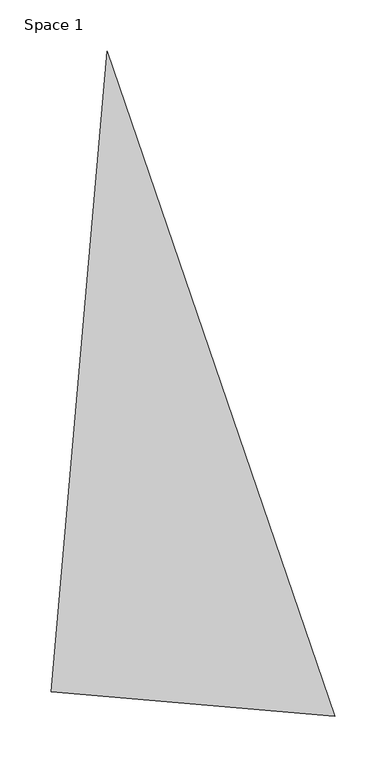
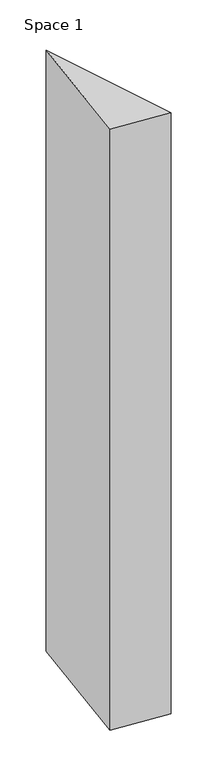
"""IFC4 building model written with IfcOpenShell, lengths in millimetres: proxy geometry, Space 1."""

from ifc_helpers import new_model, si_unit, point, frame_2d, origin, origin_with_axes, place, context, project, spatial, polyline, circle_curve, trimmed, segment, composite_curve, outline, extrude, source, transform, mapped, element, save


def space_1_ce7d539d(model_context):
    return source(origin(), model_context, "Body", "SweptSolid", [
        extrude(outline(composite_curve([segment(polyline([(-49811.4643156, -16324.4813217), (-49756.5523037, -15696.8341529)]), True, "CONTINUOUS"), segment(trimmed(circle_curve(frame_2d((-57151.5440345, -18598.359635)), 7943.85), [point((-49756.5523037, -15696.8341529))], [point((-49532.8505694, -16348.856866))], False, "CARTESIAN"), True, "CONTINUOUS"), segment(polyline([(-49532.8505694, -16348.856866), (-49811.4643156, -16324.4813217)]), True, "CONTINUOUS")], self_intersect=False)), origin_with_axes(), (0.0, 0.0, 1.0), 3048.0),
    ])


if __name__ == "__main__":
    model = new_model("IFC4")
    model_context = context("Model", 3, world=origin())
    ifc_project = project(units=[si_unit("LENGTHUNIT", "METRE", prefix="MILLI")], contexts=[model_context])
    site = spatial("IfcSite", under=ifc_project)
    building = spatial("IfcBuilding", under=site)
    placement = place(None, origin())
    space_1_shape = space_1_ce7d539d(model_context)
    element("IfcBuildingElementProxy", 1, Name="Space 1", ObjectType="Space 1", at=placement, inside=building, context=model_context, shape_type="MappedRepresentation", body=[
        mapped(space_1_shape, transform((0.0, 0.0, 0.0), x_axis=(1.0, 0.0, 0.0), y_axis=(0.0, 1.0, 0.0), z_axis=(0.0, 0.0, 1.0))),
    ])
    save(model, "model.ifc")

# Revit data of these elements
# Element 1 (IfcBuildingElementProxy, "Space 1")
#   Materials on its faces: "Render Material 255-255-255"
# Materials
#   "Render Material 255-255-255": class "Unassigned", colour RGB 255 255 255, transparency 0
